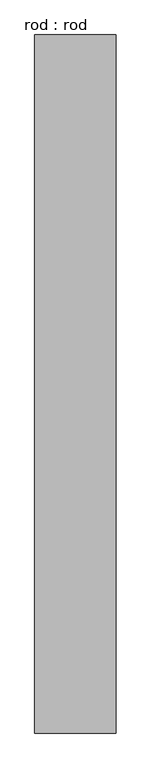
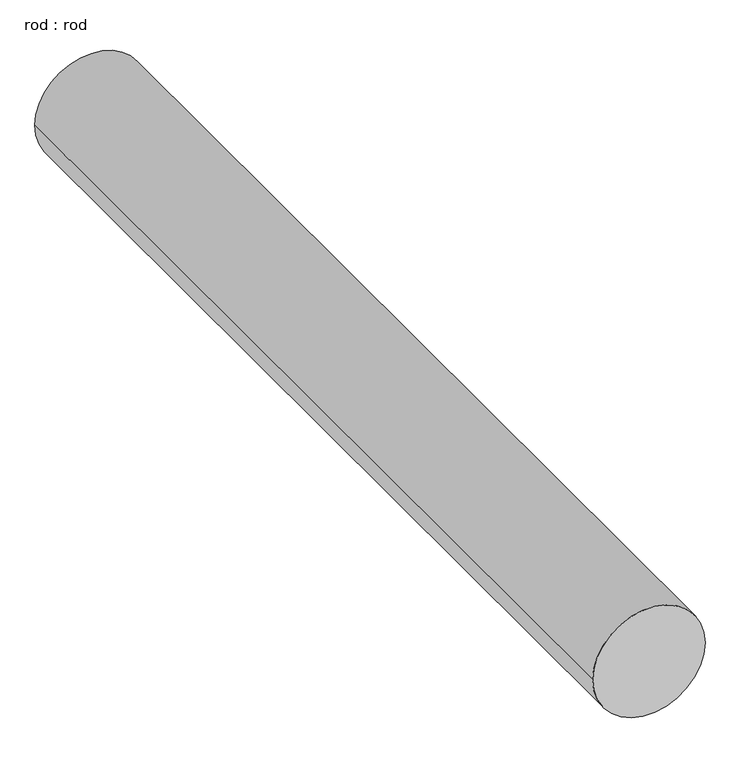
"""IFC4 building model written with IfcOpenShell, lengths in millimetres: proxy geometry, rod : rod."""

from ifc_helpers import new_model, si_unit, point, frame, frame_2d, origin, place, context, project, spatial, circle_curve, trimmed, segment, composite_curve, outline, extrude, source, transform, mapped, element, save


def rod_rod_6669fbc5(model_context):
    return source(origin(), model_context, "Body", "SweptSolid", [
        extrude(outline(composite_curve([segment(trimmed(circle_curve(frame_2d((0.0108462, 0.0)), 200.0), [point((0.0108462, 200.0))], [point((0.0108462, -200.0))], False, "CARTESIAN"), True, "CONTINUOUS"), segment(trimmed(circle_curve(frame_2d((0.0108462, 0.0)), 200.0), [point((0.0108462, -200.0))], [point((0.0108462, 200.0))], False, "CARTESIAN"), True, "CONTINUOUS")], self_intersect=False)), frame((0.0, 2373.0857582, 0.0), z_axis=(0.0, 1.0, 0.0), x_axis=(0.0, 0.0, 1.0)), (0.0, 0.0, 1.0), 3439.2857143),
    ])


if __name__ == "__main__":
    model = new_model("IFC4")
    model_context = context("Model", 3, world=origin())
    ifc_project = project(units=[si_unit("LENGTHUNIT", "METRE", prefix="MILLI")], contexts=[model_context])
    site = spatial("IfcSite", under=ifc_project)
    building = spatial("IfcBuilding", under=site)
    placement = place(None, origin())
    rod_rod_shape = rod_rod_6669fbc5(model_context)
    element("IfcBuildingElementProxy", 1, Name="rod : rod", ObjectType="rod : rod", at=placement, inside=building, context=model_context, shape_type="MappedRepresentation", body=[
        mapped(rod_rod_shape, transform((0.0, 0.0, 0.0), x_axis=(1.0, 0.0, 0.0), y_axis=(0.0, 1.0, 0.0), z_axis=(0.0, 0.0, 1.0))),
    ])
    save(model, "model.ifc")

# Revit data of these elements
# Type "rod : rod"
#   Default Elevation = 0
